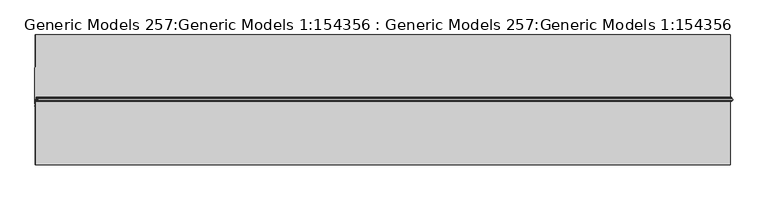
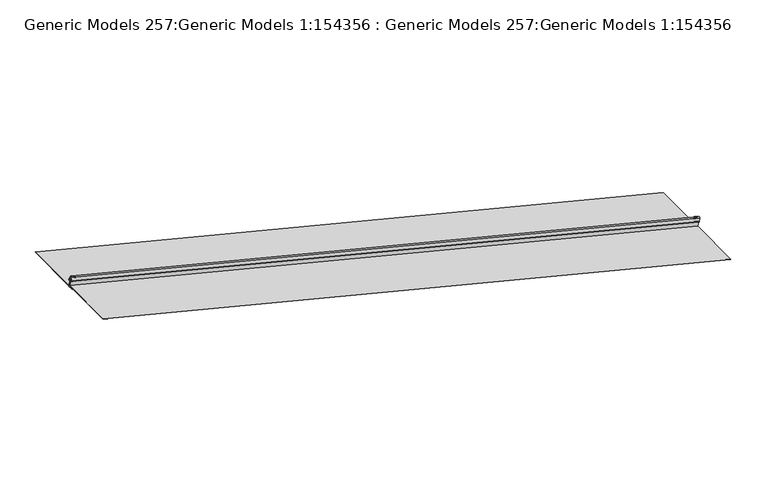
"""IFC4 building model written with IfcOpenShell, lengths in millimetres: proxy geometry, Generic Models 257:Generic Models 1:154356 : Generic Models 257:Generic Models 1:154356."""

import ifcopenshell
import ifcopenshell.guid

model = None  # the IFC model being written
_history = None  # IfcOwnerHistory: only IFC2X3 demands one
_inside = {}  # id of a spatial element -> (the spatial element, [elements in it])
_under = {}  # id of a project, library or spatial element -> (it, [spatial elements below it])
_declared = {}  # id of a project -> (the project, [libraries it declares])
_typed = {}  # id of a type object -> (the type object, [elements of that type])
_made_of = {}  # id of a material, layer set ... -> (it, [elements and type objects made of it])


def new_model(schema):
    """Start an empty IFC model of exactly this schema.

    Asked for "IFC4X3", IfcOpenShell would pick the latest addendum, in which some entities
    have other attributes; the version numbers below select the first issue.
    IFC2X3 requires an IfcOwnerHistory on every rooted entity: one is made here for all.
    """
    global model, _history
    if schema == "IFC4X3":
        model = ifcopenshell.file(schema_version=(4, 3, 0, 0))
    else:
        model = ifcopenshell.file(schema=schema)
    _inside.clear()
    _under.clear()
    _declared.clear()
    _typed.clear()
    _made_of.clear()
    _history = None
    if model.schema == "IFC2X3":
        org = make("IfcOrganization", Name="unknown")
        user = make(
            "IfcPersonAndOrganization",
            ThePerson=make("IfcPerson", FamilyName="unknown"),
            TheOrganization=org,
        )
        app = make(
            "IfcApplication",
            ApplicationDeveloper=org,
            Version="unknown",
            ApplicationFullName="unknown",
            ApplicationIdentifier="unknown",
        )
        _history = make(
            "IfcOwnerHistory",
            OwningUser=user,
            OwningApplication=app,
            ChangeAction="ADDED",
            CreationDate=0,
        )
    return model


def make(cls, **values):
    """One entity of the class cls with the attributes given. An attribute that is None is left unset."""
    return model.create_entity(
        cls, **{name: value for name, value in values.items() if value is not None}
    )


def rooted(cls, **values):
    """An entity with a GlobalId (a new one), such as an element, a storey or a relation."""
    return make(cls, GlobalId=ifcopenshell.guid.new(), OwnerHistory=_history, **values)


def si_unit(unit_type, name, prefix=None):
    """IfcSIUnit, for example si_unit("LENGTHUNIT", "METRE", prefix="MILLI")."""
    return make("IfcSIUnit", UnitType=unit_type, Prefix=prefix, Name=name)


def assignment(units):
    """IfcUnitAssignment: the units of a project."""
    return None if units is None else make("IfcUnitAssignment", Units=units)


def point(xyz):
    """IfcCartesianPoint."""
    return None if xyz is None else make("IfcCartesianPoint", Coordinates=xyz)


def direction(xyz):
    """IfcDirection."""
    return None if xyz is None else make("IfcDirection", DirectionRatios=xyz)


def frame(location, z_axis=None, x_axis=None):
    """IfcAxis2Placement3D, a coordinate frame: its origin and axes. An axis left out is left unset."""
    return make(
        "IfcAxis2Placement3D",
        Location=point(location),
        Axis=direction(z_axis),
        RefDirection=direction(x_axis),
    )


def frame_2d(location, x_axis=None):
    """IfcAxis2Placement2D, a coordinate frame in the plane: its origin and x axis."""
    return make(
        "IfcAxis2Placement2D", Location=point(location), RefDirection=direction(x_axis)
    )


def origin():
    """The frame at (0, 0, 0) with its axes left unset."""
    return frame((0.0, 0.0, 0.0))


def place(relative_to, where):
    """IfcLocalPlacement: puts the frame where relative to a parent placement (None: the world)."""
    return make(
        "IfcLocalPlacement", PlacementRelTo=relative_to, RelativePlacement=where
    )


def context(
    kind, dimensions, precision=None, world=None, true_north=None, identifier=None
):
    """IfcGeometricRepresentationContext, for example the 3D "Model" context."""
    return make(
        "IfcGeometricRepresentationContext",
        ContextIdentifier=identifier,
        ContextType=kind,
        CoordinateSpaceDimension=dimensions,
        Precision=precision,
        WorldCoordinateSystem=world,
        TrueNorth=true_north,
    )


def project(units=None, contexts=None):
    """IfcProject with its units and contexts."""
    return rooted(
        "IfcProject",
        Name="project",
        RepresentationContexts=contexts,
        UnitsInContext=assignment(units),
    )


def spatial(cls, under=None, at=None, **own):
    """A site, building, storey or space (cls), placed at a placement, below another one or the project."""
    s = rooted(cls, ObjectPlacement=at, **own)
    if under is not None:
        _under.setdefault(under.id(), (under, []))[1].append(s)
    return s


def polyline(points):
    """IfcPolyline through the points."""
    return make("IfcPolyline", Points=[point(p) for p in points])


def circle_curve(where, radius):
    """IfcCircle in the frame where."""
    return make("IfcCircle", Position=where, Radius=radius)


def trimmed(basis, trim1, trim2, sense, master):
    """IfcTrimmedCurve: the piece of a basis curve between two trims."""
    return make(
        "IfcTrimmedCurve",
        BasisCurve=basis,
        Trim1=trim1,
        Trim2=trim2,
        SenseAgreement=sense,
        MasterRepresentation=master,
    )


def segment(curve, same_sense, transition):
    """IfcCompositeCurveSegment."""
    return make(
        "IfcCompositeCurveSegment",
        Transition=transition,
        SameSense=same_sense,
        ParentCurve=curve,
    )


def composite_curve(segments, self_intersect=None):
    """IfcCompositeCurve: segments joined end to end."""
    return make("IfcCompositeCurve", Segments=segments, SelfIntersect=self_intersect)


def outline(outer, holes=None, kind="AREA"):
    """IfcArbitraryClosedProfileDef: a profile drawn as a closed curve; with holes, ...WithVoids."""
    if holes is None:
        return make("IfcArbitraryClosedProfileDef", ProfileType=kind, OuterCurve=outer)
    return make(
        "IfcArbitraryProfileDefWithVoids",
        ProfileType=kind,
        OuterCurve=outer,
        InnerCurves=holes,
    )


def extrude(swept, where, along, depth):
    """IfcExtrudedAreaSolid: the profile swept, set in the frame where, extruded along a direction by depth."""
    return make(
        "IfcExtrudedAreaSolid",
        SweptArea=swept,
        Position=where,
        ExtrudedDirection=direction(along),
        Depth=depth,
    )


def shape(context_of_items, identifier, shape_type, items):
    """IfcShapeRepresentation: the items that make up one representation, for example the "Body"."""
    return make(
        "IfcShapeRepresentation",
        ContextOfItems=context_of_items,
        RepresentationIdentifier=identifier,
        RepresentationType=shape_type,
        Items=items,
    )


def source(mapping_origin, context_of_items, identifier, shape_type, items):
    """IfcRepresentationMap: a shape defined once, which mapped items show again and again."""
    return make(
        "IfcRepresentationMap",
        MappingOrigin=mapping_origin,
        MappedRepresentation=shape(context_of_items, identifier, shape_type, items),
    )


def transform(
    local_origin,
    x_axis=None,
    y_axis=None,
    z_axis=None,
    scale=None,
    scale2=None,
    scale3=None,
    uniform=True,
):
    """IfcCartesianTransformationOperator3D, or its non-uniform kind. x_axis, y_axis, z_axis: its Axis1, 2, 3."""
    if uniform:
        return make(
            "IfcCartesianTransformationOperator3D",
            Axis1=direction(x_axis),
            Axis2=direction(y_axis),
            LocalOrigin=point(local_origin),
            Scale=scale,
            Axis3=direction(z_axis),
        )
    return make(
        "IfcCartesianTransformationOperator3DnonUniform",
        Axis1=direction(x_axis),
        Axis2=direction(y_axis),
        LocalOrigin=point(local_origin),
        Scale=scale,
        Axis3=direction(z_axis),
        Scale2=scale2,
        Scale3=scale3,
    )


def mapped(mapping_source, mapping_target):
    """IfcMappedItem: shows the shape of a source again, moved by a transform."""
    return make(
        "IfcMappedItem", MappingSource=mapping_source, MappingTarget=mapping_target
    )


def made_of(thing, what):
    """Note that an element or type object is made of a material, layer set ...; save() writes the relation."""
    if what is not None:
        _made_of.setdefault(what.id(), (what, []))[1].append(thing)
    return thing


def element(
    cls,
    number,
    at=None,
    inside=None,
    cuts=None,
    type_object=None,
    material=None,
    context=None,
    identifier="Body",
    shape_type=None,
    held_by="IfcProductDefinitionShape",
    body=None,
    shapes=None,
    **own,
):
    """One element of the class cls, such as IfcWall. Its Tag is "e" and its number.

    at: its placement. inside: the storey or other place that contains it. cuts: it is an
    opening in that element (IfcRelVoidsElement). A single representation is given by context,
    identifier, shape_type and body (its items); several are given by shapes. held_by: the class
    of the entity that holds the representations. save() writes the other relations.
    """
    e = rooted(cls, Tag="e%d" % number, ObjectPlacement=at, **own)
    if body is not None:
        shapes = [shape(context, identifier, shape_type, body)]
    if shapes is not None:
        e.Representation = make(held_by, Representations=shapes)
    if inside is not None:
        _inside.setdefault(inside.id(), (inside, []))[1].append(e)
    if cuts is not None:
        rooted(
            "IfcRelVoidsElement", RelatingBuildingElement=cuts, RelatedOpeningElement=e
        )
    if type_object is not None:
        _typed.setdefault(type_object.id(), (type_object, []))[1].append(e)
    return made_of(e, material)


def aggregate(whole, parts):
    """IfcRelAggregates: a whole, such as a stair, and the parts it consists of."""
    return rooted("IfcRelAggregates", RelatingObject=whole, RelatedObjects=parts)


def save(model, path):
    """Write the relations noted so far, then the file.

    IfcRelAggregates (storeys below a building ...), IfcRelContainedInSpatialStructure (elements
    in a storey), IfcRelDefinesByType, IfcRelAssociatesMaterial and IfcRelDeclares: one each for
    every whole, place, type object, material and project.
    """
    for whole, parts in _under.values():
        aggregate(whole, parts)
    for where, things in _inside.values():
        rooted(
            "IfcRelContainedInSpatialStructure",
            RelatedElements=things,
            RelatingStructure=where,
        )
    for kind, things in _typed.values():
        rooted("IfcRelDefinesByType", RelatedObjects=things, RelatingType=kind)
    for what, things in _made_of.values():
        rooted("IfcRelAssociatesMaterial", RelatedObjects=things, RelatingMaterial=what)
    for by, libraries in _declared.values():
        rooted("IfcRelDeclares", RelatingContext=by, RelatedDefinitions=libraries)
    model.write(path)


def plane_surface(at):
    """IfcPlane: the flat surface through the origin of the frame at, square to its z axis."""
    return make("IfcPlane", Position=at)


def cylinder_surface(at, radius):
    """IfcCylindricalSurface: all points at the distance radius from the z axis of the frame at."""
    return make("IfcCylindricalSurface", Position=at, Radius=radius)


def revolved_surface(curve, axis_point, axis_direction):
    """IfcSurfaceOfRevolution: the curve turned about the line through axis_point along axis_direction."""
    return make(
        "IfcSurfaceOfRevolution",
        SweptCurve=make("IfcArbitraryOpenProfileDef", ProfileType="CURVE", Curve=curve),
        AxisPosition=make("IfcAxis1Placement", Location=point(axis_point), Axis=direction(axis_direction)),
    )


def advanced_brep(points, edges, surfaces, faces):
    """IfcAdvancedBrep: a solid bounded by faces that lie on surfaces and meet in shared edges.

    An edge is (start, end): straight between two places in points (the first is 0);
    or (start, end, curve); or (start, end, curve, False) where it runs against its curve.
    A face is (place in surfaces, loops), or (place, loops, False) where it looks against
    its surface's normal. A loop lists edges by number (the first is 1), with a minus sign
    where the edge is run from its end to its start. The first loop is the outer one.
    """
    corners = [point(p) for p in points]
    vertices = [make("IfcVertexPoint", VertexGeometry=c) for c in corners]
    made = []
    for start, end, *more in edges:
        made.append(
            make(
                "IfcEdgeCurve",
                EdgeStart=vertices[start],
                EdgeEnd=vertices[end],
                EdgeGeometry=more[0] if more else make("IfcPolyline", Points=[corners[start], corners[end]]),
                SameSense=more[1] if len(more) > 1 else True,
            )
        )
    hull = []
    for where, loops, *sense in faces:
        bounds = []
        for j, loop in enumerate(loops):
            ring = [make("IfcOrientedEdge", EdgeElement=made[abs(k) - 1], Orientation=k > 0) for k in loop]
            bounds.append(
                make(
                    "IfcFaceOuterBound" if j == 0 else "IfcFaceBound",
                    Bound=make("IfcEdgeLoop", EdgeList=ring),
                    Orientation=True,
                )
            )
        hull.append(make("IfcAdvancedFace", Bounds=bounds, FaceSurface=surfaces[where], SameSense=sense[0] if sense else True))
    return make("IfcAdvancedBrep", Outer=make("IfcClosedShell", CfsFaces=hull))


def generic_models_257_generic_models_1_154356_generic_models_a5a0b37f(model_context):
    return source(origin(), model_context, "Body", "SolidModel", [
        extrude(outline(composite_curve([segment(trimmed(circle_curve(frame_2d((-3.5496379, 0.0)), 3.5496379), [point((0.0, 0.0))], [point((-4.8615212, -3.2983165))], False, "CARTESIAN"), True, "CONTINUOUS"), segment(polyline([(-4.8615212, -3.2983165), (-14.9309143, 0.7067172)]), True, "CONTINUOUS"), segment(trimmed(circle_curve(frame_2d((-13.4600367, 3.8026836)), 3.4276069), [point((-14.9309143, 0.7067172))], [point((-14.9442984, 6.8922559))], False, "CARTESIAN"), True, "CONTINUOUS"), segment(trimmed(circle_curve(frame_2d((6.6820881, -74.8850549)), 84.5885876), [point((-14.9442984, 6.8922559))], [point((-3.3514748, 9.106354))], False, "CARTESIAN"), True, "CONTINUOUS"), segment(trimmed(circle_curve(frame_2d((-2.9002937, 6.7043507)), 2.4440099), [point((-3.3514748, 9.106354))], [point((-0.5455984, 7.3590216))], False, "CARTESIAN"), True, "CONTINUOUS"), segment(polyline([(-0.5455984, 7.3590216), (14.3551521, 7.6191152), (15.7935498, 213.3452671), (16.6687642, 213.3452671), (15.2249456, 6.8437836), (-0.0769429, 6.5766881)]), True, "CONTINUOUS"), segment(trimmed(circle_curve(frame_2d((-0.1000536, 8.0144412)), 1.4379388), [point((-0.0769429, 6.5766881))], [point((-1.4036804, 7.4076254))], False, "CARTESIAN"), True, "CONTINUOUS"), segment(trimmed(circle_curve(frame_2d((-2.9002937, 6.7043507)), 1.6536163), [point((-1.4036804, 7.4076254))], [point((-3.229013, 8.3249649))], True, "CARTESIAN"), True, "CONTINUOUS"), segment(trimmed(circle_curve(frame_2d((6.6820881, -74.8850549)), 83.798194), [point((-3.229013, 8.3249649))], [point((-14.6650356, 6.1485038))], True, "CARTESIAN"), True, "CONTINUOUS"), segment(trimmed(circle_curve(frame_2d((-13.4600367, 3.8026836)), 2.6372134), [point((-14.6650356, 6.1485038))], [point((-14.6133702, 1.4310352))], True, "CARTESIAN"), True, "CONTINUOUS"), segment(polyline([(-14.6133702, 1.4310352), (-4.5694058, -2.5638844)]), True, "CONTINUOUS"), segment(trimmed(circle_curve(frame_2d((-3.5496379, 0.0)), 2.7592444), [point((-4.5694058, -2.5638844))], [point((-0.7903936, 0.0))], True, "CARTESIAN"), True, "CONTINUOUS"), segment(polyline([(-0.7903936, 0.0), (0.0, 0.0)]), True, "CONTINUOUS")], self_intersect=False)), frame((1899.6486692, 5851.0567686, 6456.9896456), z_axis=(-0.9701425001453722, 0.0, 0.2425356250361718), x_axis=(-0.2425356250361718, 0.0, -0.9701425001453722)), (0.0, 0.0, 1.0), 2317.0432245),
        extrude(outline(composite_curve([segment(polyline([(-0.8341234, -0.1579888), (28.8088265, -0.1579888), (28.8088265, 10.816202), (27.3155048, 12.3095238), (27.3155048, 16.4618052), (29.2397722, 18.4066851), (29.2397722, 17.3103068), (28.1058983, 16.1579461), (28.1058983, 12.6140001), (29.5992201, 11.1206783), (29.5992201, -0.9483823), (-0.7240546, -0.9483823)]), True, "CONTINUOUS"), segment(trimmed(circle_curve(frame_2d((-0.1620961, -2.256017)), 1.4232729), [point((-0.7240546, -0.9483823))], [point((-0.8801549, -3.4848771))], True, "CARTESIAN"), True, "CONTINUOUS"), segment(trimmed(circle_curve(frame_2d((-25.317573, -64.2175917)), 65.4648763), [point((-0.8801549, -3.4848771))], [point((3.6492406, -5.5100646))], False, "CARTESIAN"), True, "CONTINUOUS"), segment(polyline([(3.6492406, -5.5100646), (3.294957, -6.2280972)]), True, "CONTINUOUS"), segment(trimmed(circle_curve(frame_2d((-25.5468296, -64.7760209)), 65.2664388), [point((3.294957, -6.2280972))], [point((-1.1996412, -4.2209018))], True, "CARTESIAN"), True, "CONTINUOUS"), segment(trimmed(circle_curve(frame_2d((0.0, -2.2809286)), 2.2809286), [point((-1.1996412, -4.2209018))], [point((-0.8341234, -0.1579888))], False, "CARTESIAN"), True, "CONTINUOUS")], self_intersect=False)), frame((1902.4293225, 5844.6883915, 6468.112259), z_axis=(-0.9701425001453219, 0.0, 0.24253562503637296), x_axis=(-0.24253562503637296, 0.0, -0.9701425001453219)), (0.0, 0.0, 1.0), 2317.0432245),
        advanced_brep(
        [(-352.3938886, 5847.9515297, 7002.2333684), (-352.0605546, 6056.8059111, 7003.5667046), (-352.2728252, 6056.8055512, 7002.7176219), (-352.6073606, 5847.1984636, 7001.3794804), (-345.7394019, 5845.9737706, 7028.8513153), (-345.6155549, 5848.5747187, 7029.3467034), (-347.6811533, 5852.4013224, 7021.0843097), (-347.7718956, 5851.7068173, 7020.7213404), (-345.6786354, 5847.8282564, 7029.0943813), (-345.7311189, 5846.763426, 7028.8844474), (1895.4682182, 5847.9515297, 6440.2678417), (1902.1309879, 5846.763426, 6466.9189207), (1902.1825775, 5847.8296193, 6467.1252789), (1900.0902112, 5851.7068173, 6458.7558137), (1900.1809535, 5852.4013224, 6459.118783), (1902.2465519, 5848.5747187, 6467.3811767), (1902.1227049, 5845.9737706, 6466.8857886), (1895.2547462, 5847.1984636, 6439.4139537), (1895.5892816, 6056.8055512, 6440.7520952), (1895.8015522, 6056.8059111, 6441.6011779)],
        [
            (0, 1),
            (1, 2),
            (2, 3),
            (3, 4),
            (4, 5, circle_curve(frame((-345.7422417, 5847.3266689, 7028.8399558), z_axis=(-0.9701425001453224, 0.0, 0.24253562503637113), x_axis=(9.974613693109772e-05, -0.9999999154310159, 0.0003989845477243258)), 1.352949)),
            (5, 6, circle_curve(frame((-340.1576776, 5910.0502978, 7051.1782123), z_axis=(0.9701425001453224, 0.0, -0.24253562503637113), x_axis=(9.974613693109772e-05, -0.9999999154310159, 0.0003989845477243258)), 65.4648763)),
            (6, 7),
            (7, 8, circle_curve(frame((-340.1850009, 5909.773837, 7051.0689192), z_axis=(-0.9701425001453224, 0.0, 0.24253562503637113), x_axis=(9.974613693109772e-05, -0.9999999154310159, 0.0003989845477243258)), 65.9569199)),
            (8, 9, circle_curve(frame((-345.7253542, 5847.3129989, 7028.9075061), z_axis=(0.9701425001453224, 0.0, -0.24253562503637113), x_axis=(9.974613693109772e-05, -0.9999999154310159, 0.0003989845477243258)), 0.5500866)),
            (9, 0),
            (10, 11),
            (11, 12, circle_curve(frame((1902.1367526, 5847.3129989, 6466.9419794), z_axis=(-0.9701425001453224, 0.0, 0.24253562503637113), x_axis=(9.974613693109772e-05, -0.9999999154310159, 0.0003989845477243258)), 0.5500866)),
            (12, 13, circle_curve(frame((1907.6771059, 5909.773837, 6489.1033925), z_axis=(0.9701425001453224, 0.0, -0.24253562503637113), x_axis=(9.974613693109772e-05, -0.9999999154310159, 0.0003989845477243258)), 65.9569199)),
            (13, 14),
            (14, 15, circle_curve(frame((1907.7044292, 5910.0502978, 6489.2126856), z_axis=(-0.9701425001453224, 0.0, 0.24253562503637113), x_axis=(9.974613693109772e-05, -0.9999999154310159, 0.0003989845477243258)), 65.4648763)),
            (15, 16, circle_curve(frame((1902.119865, 5847.3266689, 6466.8744291), z_axis=(0.9701425001453224, 0.0, -0.24253562503637113), x_axis=(9.974613693109772e-05, -0.9999999154310159, 0.0003989845477243258)), 1.352949)),
            (16, 17),
            (17, 18),
            (18, 19),
            (19, 10),
            (0, 10),
            (19, 1),
            (18, 2),
            (17, 3),
            (16, 4),
            (15, 5),
            (14, 6),
            (13, 7),
            (12, 8),
            (11, 9),
        ],
        [
            plane_surface(frame((-352.3938886, 5847.9515297, 7002.2333684), z_axis=(-0.9701425001453227, 0.0, 0.24253562503637008), x_axis=(0.0015959772010294344, 0.9999783490481954, 0.006383908804117738))),
            plane_surface(frame((1895.4682182, 5847.9515297, 6440.2678417), z_axis=(0.9701425001453227, 0.0, -0.24253562503637008), x_axis=(-0.0015959772010294344, -0.9999783490481954, -0.006383908804117738))),
            plane_surface(frame((-352.3938886, 5847.9515297, 7002.2333684), z_axis=(0.24253037390924156, -0.006580382575921991, 0.9701214956368085), x_axis=(0.9701425001453227, 0.0, -0.2425356250363701))),
            plane_surface(frame((-352.0605546, 6056.8059111, 7003.5667046), z_axis=(-9.974613706698282e-05, 0.9999999154310157, -0.0003989845482659395), x_axis=(0.9701425001453227, 0.0, -0.2425356250363701))),
            plane_surface(frame((-352.2728252, 6056.8055512, 7002.7176219), z_axis=(-0.24253037390924156, 0.006580382575919951, -0.9701214956368085), x_axis=(0.9701425001453227, 0.0, -0.2425356250363701))),
            plane_surface(frame((-352.6073606, 5847.1984636, 7001.3794804), z_axis=(-0.010479603282952775, -0.9990660761709125, -0.0419184131318062), x_axis=(0.9701425001453227, 0.0, -0.2425356250363701))),
            cylinder_surface(frame((1902.119865, 5847.3266689, 6466.8744291), z_axis=(-0.9701425001453224, 0.0, 0.24253562503637113), x_axis=(9.974613693109772e-05, -0.9999999154310159, 0.0003989845477243258)), 1.352949),
            revolved_surface(polyline([(1907.7109590685156, 5844.585427036299, 6489.238805074063), (-340.15114780205, 5844.585427036299, 7051.204331791798)]), (1907.7044292, 5910.0502978, 6489.2126856), (0.9701425001453224, 0.0, -0.24253562503637113)),
            plane_surface(frame((-347.6811533, 5852.4013224, 7021.0843097), z_axis=(-0.21352302276994556, 0.47427272607898224, -0.8540920910796425), x_axis=(0.9701425001453227, 0.0, -0.2425356250363701))),
            cylinder_surface(frame((1907.6771059, 5909.773837, 6489.1033925), z_axis=(-0.9701425001453224, 0.0, 0.24253562503637113), x_axis=(9.974613693109772e-05, -0.9999999154310159, 0.0003989845477243258)), 65.9569199),
            revolved_surface(polyline([(1902.1368074925426, 5846.76291234652, 6466.942198870171), (-345.7252993544946, 5846.76291234652, 7028.907725582024)]), (1902.1367526, 5847.3129989, 6466.9419794), (0.9701425001453224, 0.0, -0.24253562503637113)),
            plane_surface(frame((-345.7311189, 5846.763426, 7028.8844474), z_axis=(0.010479603282973706, 0.9990660761709087, 0.04191841313188993), x_axis=(0.9701425001453227, 0.0, -0.2425356250363701))),
        ],
        [
            (0, [[1, 2, 3, 4, 5, 6, 7, 8, 9, 10]]),
            (1, [[11, 12, 13, 14, 15, 16, 17, 18, 19, 20]]),
            (2, [[-1, 21, -20, 22]]),
            (3, [[-2, -22, -19, 23]]),
            (4, [[-3, -23, -18, 24]]),
            (5, [[-4, -24, -17, 25]]),
            (6, [[-5, -25, -16, 26]]),
            (7, [[-6, -26, -15, 27]]),
            (8, [[-7, -27, -14, 28]]),
            (9, [[-8, -28, -13, 29]]),
            (10, [[-9, -29, -12, 30]]),
            (11, [[-10, -30, -11, -21]]),
        ],
    ),
    ])


if __name__ == "__main__":
    model = new_model("IFC4")
    model_context = context("Model", 3, world=origin())
    ifc_project = project(units=[si_unit("LENGTHUNIT", "METRE", prefix="MILLI")], contexts=[model_context])
    site = spatial("IfcSite", under=ifc_project)
    building = spatial("IfcBuilding", under=site)
    placement = place(None, origin())
    generic_models_257_generic_models_1_154356_generic_models_shape = generic_models_257_generic_models_1_154356_generic_models_a5a0b37f(model_context)
    element("IfcBuildingElementProxy", 1, Name="Generic Models 257:Generic Models 1:154356 : Generic Models 257:Generic Models 1:154356", ObjectType="Generic Models 257:Generic Models 1:154356 : Generic Models 257:Generic Models 1:154356", at=placement, inside=building, context=model_context, shape_type="MappedRepresentation", body=[
        mapped(generic_models_257_generic_models_1_154356_generic_models_shape, transform((0.0, 0.0, 0.0), x_axis=(1.0, 0.0, 0.0), y_axis=(0.0, 1.0, 0.0), z_axis=(0.0, 0.0, 1.0))),
    ])
    save(model, "model.ifc")

# Revit data of these elements
# Type "Generic Models 257:Generic Models 1:154356 : Generic Models 257:Generic Models 1:154356"
#   NameOverride = "Generic Models 257:Generic Models 1:154356"
#   ObjectTypeOverride = "Generic Models 257:Generic Models 1"
#   Reference = "Generic Models 1"
#   Category = "Generic Models"
#   Tag = "154356"
# Element 1 (IfcBuildingElementProxy, "Generic Models 257:Generic Models 1:154356 : Generic Models 257:Generic Models 1:154356")
#   Materials on its faces: "_STANDARD SEAM METAL ROOF 21413"
# Materials
#   "_STANDARD SEAM METAL ROOF 21413": class "Unassigned", colour RGB 175 175 175, transparency 0
